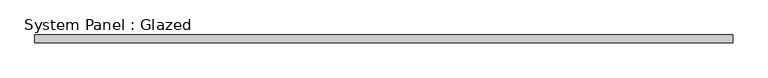
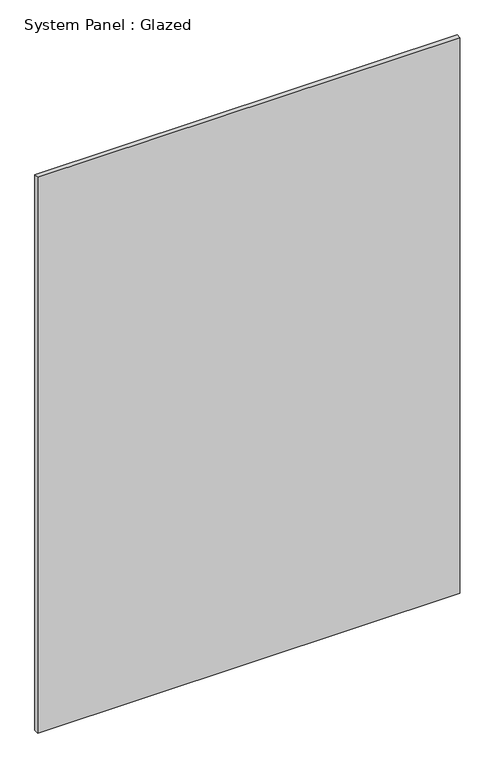
"""IFC4 building model written with IfcOpenShell, lengths in millimetres: plate geometry, System Panel : Glazed."""

from ifc_helpers import new_model, si_unit, origin, origin_with_axes, place, context, project, spatial, polyline, outline, extrude, source, transform, mapped, element, save


def system_panel_glazed_0a1ee489(model_context):
    return source(origin(), model_context, "Body", "SweptSolid", [
        extrude(outline(polyline([(1138.6652068, 24.5), (-1138.6652068, 24.5), (-1138.6652068, 49.5), (1138.6652068, 49.5), (1138.6652068, 24.5)])), origin_with_axes(), (0.0, 0.0, 1.0), 3170.0),
    ])


if __name__ == "__main__":
    model = new_model("IFC4")
    model_context = context("Model", 3, world=origin())
    ifc_project = project(units=[si_unit("LENGTHUNIT", "METRE", prefix="MILLI")], contexts=[model_context])
    site = spatial("IfcSite", under=ifc_project)
    building = spatial("IfcBuilding", under=site)
    placement = place(None, origin())
    system_panel_glazed_shape = system_panel_glazed_0a1ee489(model_context)
    element("IfcPlate", 1, ObjectType="System Panel : Glazed", at=placement, inside=building, context=model_context, shape_type="MappedRepresentation", body=[
        mapped(system_panel_glazed_shape, transform((0.0, 0.0, 0.0), x_axis=(1.0, 0.0, 0.0), y_axis=(0.0, 1.0, 0.0), z_axis=(0.0, 0.0, 1.0))),
    ])
    save(model, "model.ifc")

# Revit data of these elements
# Type "System Panel : Glazed"
#   Construction Type Id = "GSP4R"
#   Analytic Construction = "1/8 in Pilkington single glazing"
#   Visual Light Transmittance = 0.9
#   Solar Heat Gain Coefficient = 0.86
#   Heat Transfer Coefficient (U) = 6.7069 W/(m²·K)
#   Define Thermal Properties by = 1
# Element 1 (IfcPlate, "System Panel : Glazed")
#   Materials on its faces: "Glass"
# Materials
#   "Glass": class "Glass", colour RGB 245 245 243, transparency 1, Description = "Soda Lime Glass", Cost = 0
